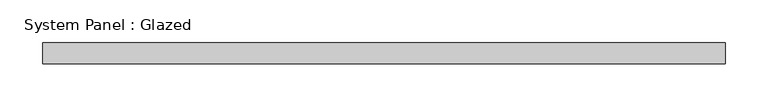
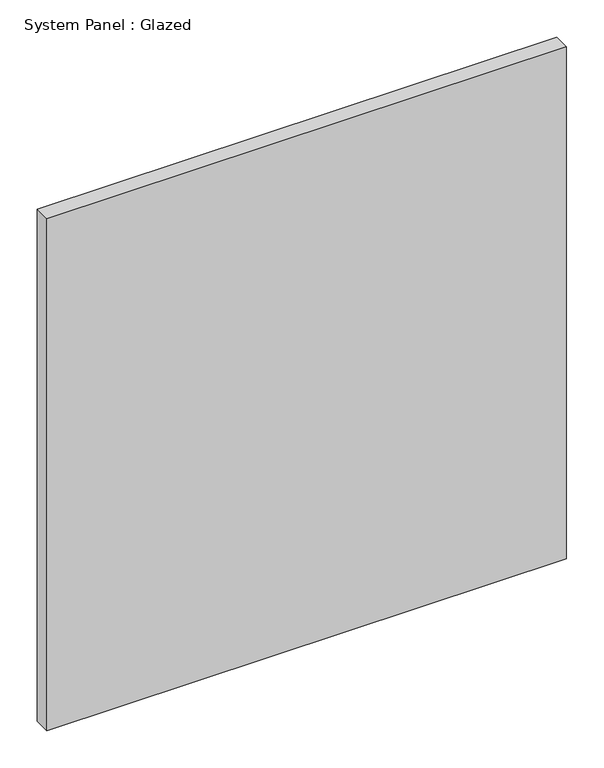
"""IFC4 building model written with IfcOpenShell, lengths in millimetres: plate geometry, System Panel : Glazed."""

from ifc_helpers import new_model, si_unit, origin, origin_with_axes, place, context, project, spatial, polyline, outline, extrude, source, transform, mapped, element, save


def system_panel_glazed_f3b9a5c0(model_context):
    return source(origin(), model_context, "Body", "SweptSolid", [
        extrude(outline(polyline([(400.0, 24.5), (-400.0, 24.5), (-400.0, 49.5), (400.0, 49.5), (400.0, 24.5)])), origin_with_axes(), (0.0, 0.0, 1.0), 833.3333333),
    ])


if __name__ == "__main__":
    model = new_model("IFC4")
    model_context = context("Model", 3, world=origin())
    ifc_project = project(units=[si_unit("LENGTHUNIT", "METRE", prefix="MILLI")], contexts=[model_context])
    site = spatial("IfcSite", under=ifc_project)
    building = spatial("IfcBuilding", under=site)
    placement = place(None, origin())
    system_panel_glazed_shape = system_panel_glazed_f3b9a5c0(model_context)
    element("IfcPlate", 1, ObjectType="System Panel : Glazed", at=placement, inside=building, context=model_context, shape_type="MappedRepresentation", body=[
        mapped(system_panel_glazed_shape, transform((0.0, 0.0, 0.0), x_axis=(1.0, 0.0, 0.0), y_axis=(0.0, 1.0, 0.0), z_axis=(0.0, 0.0, 1.0))),
    ])
    save(model, "model.ifc")

# Revit data of these elements
# Element 1 (IfcPlate, "System Panel : Glazed")
#   Materials on its faces: "Glass"
# Materials
#   "Glass": class "Glass", colour RGB 218 227 224, transparency 0.85, Description = "Soda Lime Glass", Cost = 0
